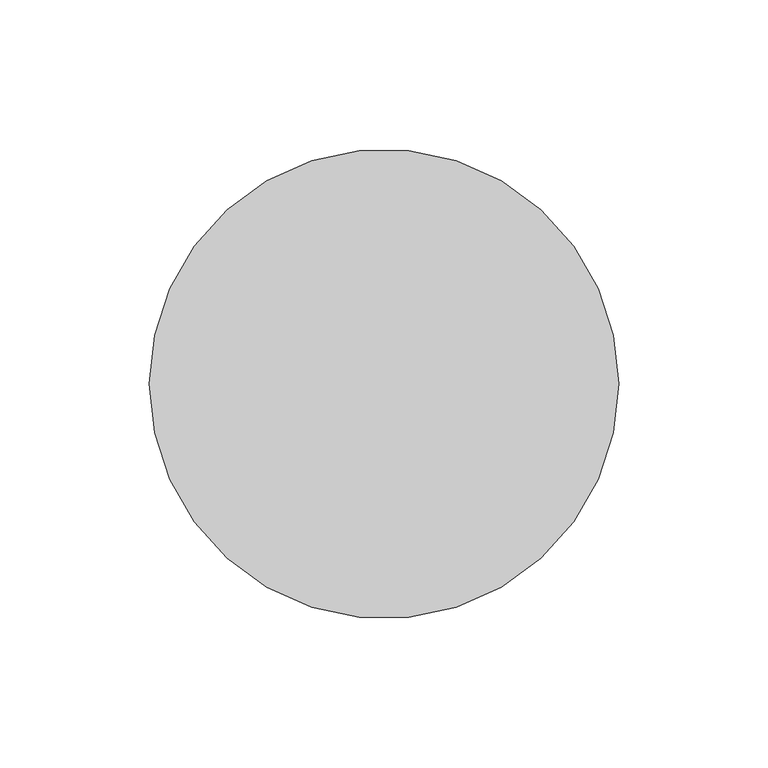
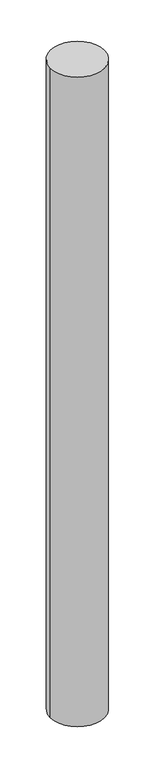
"""IFC4 building model written with IfcOpenShell, lengths in millimetres: proxy geometry, NLRS_71_GM_WPB_afschermpaal aardebaan_gen_rsf : afschermpaal aardebaan dxl 159x2000mm."""

import ifcopenshell
import ifcopenshell.guid

model = None  # the IFC model being written
_history = None  # IfcOwnerHistory: only IFC2X3 demands one
_inside = {}  # id of a spatial element -> (the spatial element, [elements in it])
_under = {}  # id of a project, library or spatial element -> (it, [spatial elements below it])
_declared = {}  # id of a project -> (the project, [libraries it declares])
_typed = {}  # id of a type object -> (the type object, [elements of that type])
_made_of = {}  # id of a material, layer set ... -> (it, [elements and type objects made of it])


def new_model(schema):
    """Start an empty IFC model of exactly this schema.

    Asked for "IFC4X3", IfcOpenShell would pick the latest addendum, in which some entities
    have other attributes; the version numbers below select the first issue.
    IFC2X3 requires an IfcOwnerHistory on every rooted entity: one is made here for all.
    """
    global model, _history
    if schema == "IFC4X3":
        model = ifcopenshell.file(schema_version=(4, 3, 0, 0))
    else:
        model = ifcopenshell.file(schema=schema)
    _inside.clear()
    _under.clear()
    _declared.clear()
    _typed.clear()
    _made_of.clear()
    _history = None
    if model.schema == "IFC2X3":
        org = make("IfcOrganization", Name="unknown")
        user = make(
            "IfcPersonAndOrganization",
            ThePerson=make("IfcPerson", FamilyName="unknown"),
            TheOrganization=org,
        )
        app = make(
            "IfcApplication",
            ApplicationDeveloper=org,
            Version="unknown",
            ApplicationFullName="unknown",
            ApplicationIdentifier="unknown",
        )
        _history = make(
            "IfcOwnerHistory",
            OwningUser=user,
            OwningApplication=app,
            ChangeAction="ADDED",
            CreationDate=0,
        )
    return model


def make(cls, **values):
    """One entity of the class cls with the attributes given. An attribute that is None is left unset."""
    return model.create_entity(
        cls, **{name: value for name, value in values.items() if value is not None}
    )


def rooted(cls, **values):
    """An entity with a GlobalId (a new one), such as an element, a storey or a relation."""
    return make(cls, GlobalId=ifcopenshell.guid.new(), OwnerHistory=_history, **values)


def si_unit(unit_type, name, prefix=None):
    """IfcSIUnit, for example si_unit("LENGTHUNIT", "METRE", prefix="MILLI")."""
    return make("IfcSIUnit", UnitType=unit_type, Prefix=prefix, Name=name)


def assignment(units):
    """IfcUnitAssignment: the units of a project."""
    return None if units is None else make("IfcUnitAssignment", Units=units)


def point(xyz):
    """IfcCartesianPoint."""
    return None if xyz is None else make("IfcCartesianPoint", Coordinates=xyz)


def direction(xyz):
    """IfcDirection."""
    return None if xyz is None else make("IfcDirection", DirectionRatios=xyz)


def frame(location, z_axis=None, x_axis=None):
    """IfcAxis2Placement3D, a coordinate frame: its origin and axes. An axis left out is left unset."""
    return make(
        "IfcAxis2Placement3D",
        Location=point(location),
        Axis=direction(z_axis),
        RefDirection=direction(x_axis),
    )


def frame_2d(location, x_axis=None):
    """IfcAxis2Placement2D, a coordinate frame in the plane: its origin and x axis."""
    return make(
        "IfcAxis2Placement2D", Location=point(location), RefDirection=direction(x_axis)
    )


def origin():
    """The frame at (0, 0, 0) with its axes left unset."""
    return frame((0.0, 0.0, 0.0))


def place(relative_to, where):
    """IfcLocalPlacement: puts the frame where relative to a parent placement (None: the world)."""
    return make(
        "IfcLocalPlacement", PlacementRelTo=relative_to, RelativePlacement=where
    )


def context(
    kind, dimensions, precision=None, world=None, true_north=None, identifier=None
):
    """IfcGeometricRepresentationContext, for example the 3D "Model" context."""
    return make(
        "IfcGeometricRepresentationContext",
        ContextIdentifier=identifier,
        ContextType=kind,
        CoordinateSpaceDimension=dimensions,
        Precision=precision,
        WorldCoordinateSystem=world,
        TrueNorth=true_north,
    )


def project(units=None, contexts=None):
    """IfcProject with its units and contexts."""
    return rooted(
        "IfcProject",
        Name="project",
        RepresentationContexts=contexts,
        UnitsInContext=assignment(units),
    )


def spatial(cls, under=None, at=None, **own):
    """A site, building, storey or space (cls), placed at a placement, below another one or the project."""
    s = rooted(cls, ObjectPlacement=at, **own)
    if under is not None:
        _under.setdefault(under.id(), (under, []))[1].append(s)
    return s


def circle_curve(where, radius):
    """IfcCircle in the frame where."""
    return make("IfcCircle", Position=where, Radius=radius)


def trimmed(basis, trim1, trim2, sense, master):
    """IfcTrimmedCurve: the piece of a basis curve between two trims."""
    return make(
        "IfcTrimmedCurve",
        BasisCurve=basis,
        Trim1=trim1,
        Trim2=trim2,
        SenseAgreement=sense,
        MasterRepresentation=master,
    )


def segment(curve, same_sense, transition):
    """IfcCompositeCurveSegment."""
    return make(
        "IfcCompositeCurveSegment",
        Transition=transition,
        SameSense=same_sense,
        ParentCurve=curve,
    )


def composite_curve(segments, self_intersect=None):
    """IfcCompositeCurve: segments joined end to end."""
    return make("IfcCompositeCurve", Segments=segments, SelfIntersect=self_intersect)


def outline(outer, holes=None, kind="AREA"):
    """IfcArbitraryClosedProfileDef: a profile drawn as a closed curve; with holes, ...WithVoids."""
    if holes is None:
        return make("IfcArbitraryClosedProfileDef", ProfileType=kind, OuterCurve=outer)
    return make(
        "IfcArbitraryProfileDefWithVoids",
        ProfileType=kind,
        OuterCurve=outer,
        InnerCurves=holes,
    )


def extrude(swept, where, along, depth):
    """IfcExtrudedAreaSolid: the profile swept, set in the frame where, extruded along a direction by depth."""
    return make(
        "IfcExtrudedAreaSolid",
        SweptArea=swept,
        Position=where,
        ExtrudedDirection=direction(along),
        Depth=depth,
    )


def shape(context_of_items, identifier, shape_type, items):
    """IfcShapeRepresentation: the items that make up one representation, for example the "Body"."""
    return make(
        "IfcShapeRepresentation",
        ContextOfItems=context_of_items,
        RepresentationIdentifier=identifier,
        RepresentationType=shape_type,
        Items=items,
    )


def source(mapping_origin, context_of_items, identifier, shape_type, items):
    """IfcRepresentationMap: a shape defined once, which mapped items show again and again."""
    return make(
        "IfcRepresentationMap",
        MappingOrigin=mapping_origin,
        MappedRepresentation=shape(context_of_items, identifier, shape_type, items),
    )


def transform(
    local_origin,
    x_axis=None,
    y_axis=None,
    z_axis=None,
    scale=None,
    scale2=None,
    scale3=None,
    uniform=True,
):
    """IfcCartesianTransformationOperator3D, or its non-uniform kind. x_axis, y_axis, z_axis: its Axis1, 2, 3."""
    if uniform:
        return make(
            "IfcCartesianTransformationOperator3D",
            Axis1=direction(x_axis),
            Axis2=direction(y_axis),
            LocalOrigin=point(local_origin),
            Scale=scale,
            Axis3=direction(z_axis),
        )
    return make(
        "IfcCartesianTransformationOperator3DnonUniform",
        Axis1=direction(x_axis),
        Axis2=direction(y_axis),
        LocalOrigin=point(local_origin),
        Scale=scale,
        Axis3=direction(z_axis),
        Scale2=scale2,
        Scale3=scale3,
    )


def mapped(mapping_source, mapping_target):
    """IfcMappedItem: shows the shape of a source again, moved by a transform."""
    return make(
        "IfcMappedItem", MappingSource=mapping_source, MappingTarget=mapping_target
    )


def made_of(thing, what):
    """Note that an element or type object is made of a material, layer set ...; save() writes the relation."""
    if what is not None:
        _made_of.setdefault(what.id(), (what, []))[1].append(thing)
    return thing


def element(
    cls,
    number,
    at=None,
    inside=None,
    cuts=None,
    type_object=None,
    material=None,
    context=None,
    identifier="Body",
    shape_type=None,
    held_by="IfcProductDefinitionShape",
    body=None,
    shapes=None,
    **own,
):
    """One element of the class cls, such as IfcWall. Its Tag is "e" and its number.

    at: its placement. inside: the storey or other place that contains it. cuts: it is an
    opening in that element (IfcRelVoidsElement). A single representation is given by context,
    identifier, shape_type and body (its items); several are given by shapes. held_by: the class
    of the entity that holds the representations. save() writes the other relations.
    """
    e = rooted(cls, Tag="e%d" % number, ObjectPlacement=at, **own)
    if body is not None:
        shapes = [shape(context, identifier, shape_type, body)]
    if shapes is not None:
        e.Representation = make(held_by, Representations=shapes)
    if inside is not None:
        _inside.setdefault(inside.id(), (inside, []))[1].append(e)
    if cuts is not None:
        rooted(
            "IfcRelVoidsElement", RelatingBuildingElement=cuts, RelatedOpeningElement=e
        )
    if type_object is not None:
        _typed.setdefault(type_object.id(), (type_object, []))[1].append(e)
    return made_of(e, material)


def aggregate(whole, parts):
    """IfcRelAggregates: a whole, such as a stair, and the parts it consists of."""
    return rooted("IfcRelAggregates", RelatingObject=whole, RelatedObjects=parts)


def save(model, path):
    """Write the relations noted so far, then the file.

    IfcRelAggregates (storeys below a building ...), IfcRelContainedInSpatialStructure (elements
    in a storey), IfcRelDefinesByType, IfcRelAssociatesMaterial and IfcRelDeclares: one each for
    every whole, place, type object, material and project.
    """
    for whole, parts in _under.values():
        aggregate(whole, parts)
    for where, things in _inside.values():
        rooted(
            "IfcRelContainedInSpatialStructure",
            RelatedElements=things,
            RelatingStructure=where,
        )
    for kind, things in _typed.values():
        rooted("IfcRelDefinesByType", RelatedObjects=things, RelatingType=kind)
    for what, things in _made_of.values():
        rooted("IfcRelAssociatesMaterial", RelatedObjects=things, RelatingMaterial=what)
    for by, libraries in _declared.values():
        rooted("IfcRelDeclares", RelatingContext=by, RelatedDefinitions=libraries)
    model.write(path)


def generic_models_0e34d4cd(model_context):
    return source(origin(), model_context, "Body", "SweptSolid", [
        extrude(outline(composite_curve([segment(trimmed(circle_curve(frame_2d((1.2, 75.0)), 78.5), [point((-77.3, 75.0))], [point((79.7, 75.0))], False, "CARTESIAN"), True, "CONTINUOUS"), segment(trimmed(circle_curve(frame_2d((1.2, 75.0)), 78.5), [point((79.7, 75.0))], [point((-77.3, 75.0))], False, "CARTESIAN"), True, "CONTINUOUS")], self_intersect=False)), frame((0.0, 0.0, -1000.0), z_axis=(0.0, 0.0, 1.0), x_axis=(1.0, 0.0, 0.0)), (0.0, 0.0, 1.0), 2000.0),
    ])


if __name__ == "__main__":
    model = new_model("IFC4")
    model_context = context("Model", 3, world=origin())
    ifc_project = project(units=[si_unit("LENGTHUNIT", "METRE", prefix="MILLI")], contexts=[model_context])
    site = spatial("IfcSite", under=ifc_project)
    building = spatial("IfcBuilding", under=site)
    placement = place(None, origin())
    generic_models_shape = generic_models_0e34d4cd(model_context)
    element("IfcBuildingElementProxy", 1, Name="NLRS_71_GM_WPB_afschermpaal aardebaan_gen_rsf : afschermpaal aardebaan dxl 159x2000mm", ObjectType="NLRS_71_GM_WPB_afschermpaal aardebaan_gen_rsf : afschermpaal aardebaan dxl 159x2000mm", at=placement, inside=building, context=model_context, shape_type="MappedRepresentation", body=[
        mapped(generic_models_shape, transform((0.0, 0.0, 0.0), x_axis=(1.0, 0.0, 0.0), y_axis=(0.0, 1.0, 0.0), z_axis=(0.0, 0.0, 1.0))),
    ])
    save(model, "model.ifc")

# Revit data of these elements
# Project information
#   Organization Name = "RSF"
#   Organization Description = "Revit Standards Foundation"
#   Building Name = "Onderwijsmodel Bouwkundig"
#   Author = "Emiel Ham TC-lid NLRS"
#   NLRS_C_opdrachtgever_adres = "Het Zuiderkruis 17, 5215 MV, 's-Hertogenbosch"
#   NLRS_C_opdrachtgever_contactpersoon = "Bestuur RSF"
#   NLRS_C_opdrachtgever_email = "secretary@revitstandards.org"
#   NLRS_C_opdrachtgever_projectnummer = "2017.4.015"
#   NLRS_C_opdrachtgever_telefoon = "nvt"
#   NLRS_C_project_email = "tc@revitstandards.org"
#   NLRS_C_project_kadaster_gemeente = "BIMSTAD"
#   NLRS_C_project_kadaster_nummer = "3"
#   NLRS_C_project_kadaster_sectie = "D"
#   NLRS_C_project_projectleider = "Martijn de Riet"
#   NLRS_C_project_telefoon = "+316 24 28 31 75"
#   NLRS_C_leverancier_bedrijfsnaam = "Technische Commissie RSF"
#   NLRS_C_leverancier_adres = "Het Zuiderkruis 17"
#   NLRS_C_leverancier_postcode = "5215 MV"
#   NLRS_C_leverancier_plaats = "'s-Hertogenbosch"
#   NLRS_C_leverancier_telefoonnummer = "nvt"
#   NLRS_C_leverancier_fax = "nvt"
#   NLRS_C_leverancier_email = "tc@revitstandards.org"
#   Workset = "Project Info"
#   IfcSite GUID = "3a0_Qb3mb9RuT4Z3SQBcsf"
#   IfcBuilding GUID = "3a0_Qb3mb9RuT4Z3SQBcsg"
#   IfcProject GUID = "3a0_Qb3mb9RuT4Z3SQBcsh"
#   Project Issue Date = "07-10-2021"
#   Project Status = "DEFINITIEF"
#   Client Name = "Revit Standards Foundation"
#   Project Address = "Onderwijsboulevard 123\n4567 HI Bimstad"
#   Project Name = "Onderwijsmodellen NLRS"
#   Project Number = "Onderwijsmodellen"
#   BCB_ProjectFolder = "C:\\Users\\Martijn de Riet\\Downloads"
# Type "NLRS_71_GM_WPB_afschermpaal aardebaan_gen_rsf : afschermpaal aardebaan dxl 159x2000mm"
#   Type IfcGUID = "05J6pyYiTDtR2exmlhyPlb"
#   IfcName[Type] = "afschermpaal aardebaan dxl 159x2000mm"
#   IfcDescription[Type] = "verkeerspaal dxl 159x2000mm"
#   IfcObjectType[Type] = "BOLLARD"
#   IfcExportAs[Type] = "IfcGeographicElementType"
#   IfcExportType[Type] = "USERDEFINED"
#   NLRS_C_revit_versie = "2021"
#   NLRS_C_materiaal_afwerking [instance default] = ""
#   NLRS_C_content_versie = ""
#   NLRS_C_content_provider = ""
#   NLRS_C_content_handleiding = ""
#   NLRS_C_content_datum_uitgifte = ""
#   NLRS_C_content_datum_gewijzigd = ""
#   NLRS_C_content_creator = ""
#   NLRS_C_brandwerendheid_text [instance default] = ""
#   NLRS_C_brandwerendheid_EI_text [instance default] = ""
#   Model = "generiek"
#   Manufacturer = "generiek"
#   Description = "verkeerspaal dxl 159x2000mm"
#   Assembly Code = "71.10"
#   NLRS_S_gewicht [instance default] = 0.00 kg
#   NLRS_C_radius = 78.50 mm
#   NLRS_C_offset [instance default] = 0.00 mm
#   NLRS_C_hoogte = 2000.00 mm
#   NLRS_C_diepte = 1000.00 mm
#   NLRS_C_buiten [instance default] = yes
#   NLRS_C_brandwerend [instance default] = yes
#   NLRS_C_brandbaar [instance default] = yes
#   NLRS_C_materiaal = none
#   URL = ""
#   Default Elevation = 0
# Element 1 (IfcBuildingElementProxy, "NLRS_71_GM_WPB_afschermpaal aardebaan_gen_rsf : afschermpaal aardebaan dxl 159x2000mm")
#   NLRS_C_offset = 344.718 mm
